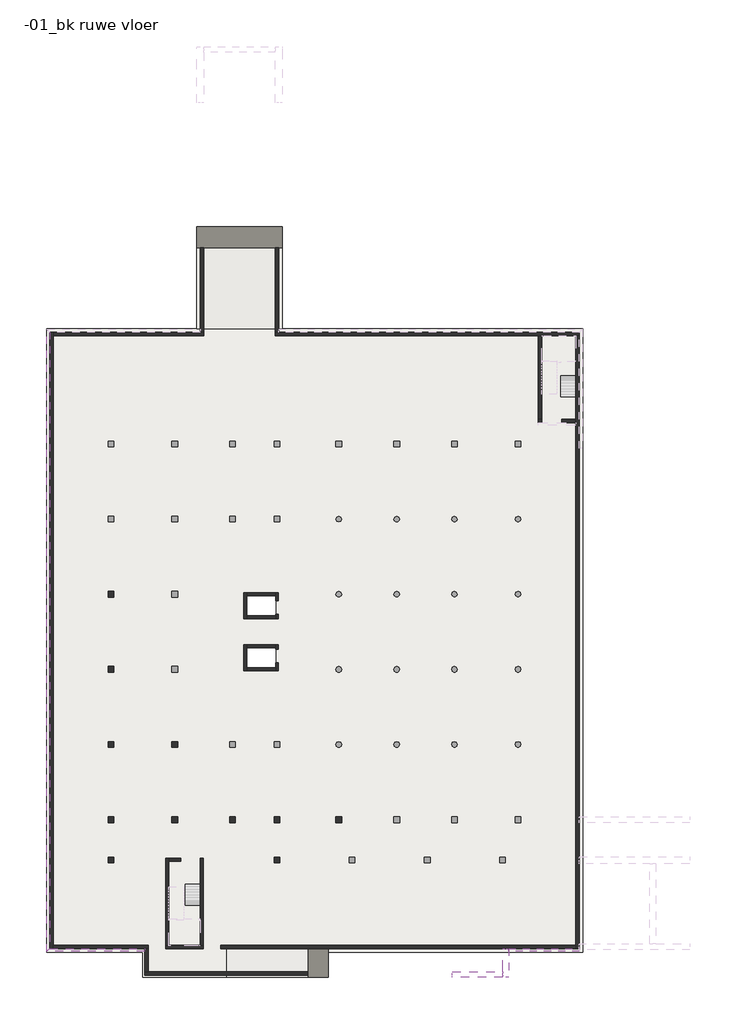
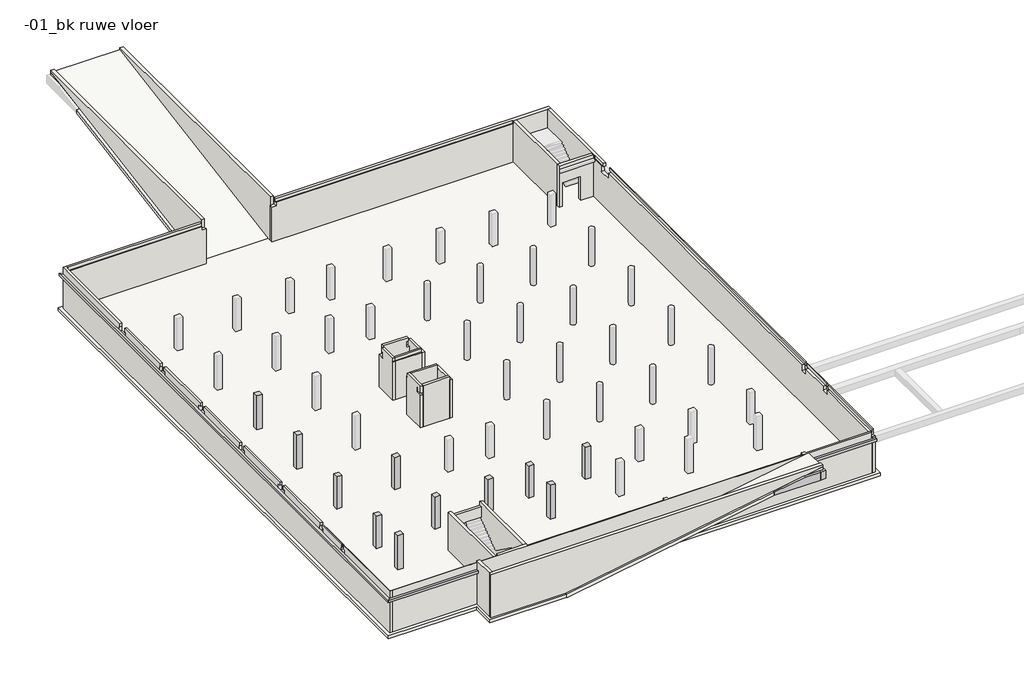
# One storey, part 1 of 2: 22 walls, 15 slabs, 11 columns, 5 beams.
"""IFC4 building model written with IfcOpenShell, lengths in millimetres."""

from ifc_helpers import new_model, si_unit, frame, origin, place, context, project, spatial, polyline, outline, extrude, faceted_brep, element, save

model = new_model("IFC4")

# Units and contexts
model_context = context("Model", 3, world=origin())
ifc_project = project(units=[si_unit("LENGTHUNIT", "METRE", prefix="MILLI")], contexts=[model_context])

# Site, building, storey
site = spatial("IfcSite", under=ifc_project)
building = spatial("IfcBuilding", under=site)
storey = spatial("IfcBuildingStorey", under=building, Name="-01_bk ruwe vloer", Elevation=-4200.0)

# Beams
placement = place(None, origin())
element("IfcBeam", 1, ObjectType="NLRS_16_SF_LIB_oplegnok beton prefab framing-CWV-MMBPC-SRP_gen_rsf : oplegnok beton prefab_gen__bxh 250x250/220", at=placement, inside=storey, context=model_context, shape_type="Brep", body=[
    faceted_brep([(6100.0, 53400.0, -970.0), (6100.0, -400.0, -970.0), (6100.0, -400.0, -750.0), (6100.0, 53400.0, -750.0), (6350.0, 53150.0, -1000.0), (6350.0, -150.0, -1000.0), (6350.0, -150.0, -750.0), (6350.0, 53150.0, -750.0)], [[[0, 1, 2, 3]], [[1, 0, 4, 5]], [[3, 2, 6, 7]], [[5, 4, 7, 6]], [[0, 3, 7, 4]], [[2, 1, 5, 6]]]),
])
element("IfcBeam", 2, ObjectType="NLRS_16_SF_LIB_oplegnok beton prefab framing-CWV-MMBPC-SRP_gen_rsf : oplegnok beton prefab_gen__bxh 250x250/220", at=placement, inside=storey, context=model_context, shape_type="Brep", body=[
    faceted_brep([(14575.0, -400.0, -750.0), (14575.0, -400.0, -970.0), (14575.0, -150.0, -1000.0), (14575.0, -150.0, -750.0), (6100.0, -400.0, -970.0), (6100.0, -400.0, -750.0), (6350.0, -150.0, -1000.0), (6350.0, -150.0, -750.0)], [[[0, 1, 2, 3]], [[4, 1, 0, 5]], [[6, 2, 1, 4]], [[7, 3, 2, 6]], [[5, 0, 3, 7]], [[5, 7, 6, 4]]]),
])
element("IfcBeam", 3, ObjectType="NLRS_16_SF_LIB_funderingsbalk beton ihwg-CWV-MMBC-SRP_gen_rsf : funderingsbalk beton ihwg_gen__bxh 500x800", at=placement, inside=storey, context=model_context, shape_type="Brep", body=[
    faceted_brep([(45545.0, -2650.0, -370.0), (46045.0, -2650.0, -370.0), (46045.0, -150.0, -370.0), (45845.0, -150.0, -370.0), (45845.0, -2450.0, -370.0), (45545.0, -2450.0, -370.0), (46045.0, -2650.0, -1170.0), (46045.0, -150.0, -1170.0), (45545.0, -2650.0, -1170.0), (45545.0, -2150.0, -1170.0), (45545.0, -150.0, -1170.0), (45545.0, -2450.0, -425.486389), (45545.0, -2150.0, -425.486389), (45545.0, -150.0, -425.486389), (45845.0, -150.0, -374.3303196), (45845.0, -2450.0, -374.3303196)], [[[0, 1, 2, 3, 4, 5]], [[1, 6, 7, 2]], [[6, 8, 9, 10, 7]], [[8, 0, 5, 11, 12, 13, 10, 9]], [[1, 0, 8, 6]], [[2, 7, 10, 13, 14, 3]], [[15, 14, 13, 12, 11]], [[14, 15, 4, 3]], [[15, 11, 5, 4]]]),
])
element("IfcBeam", 4, ObjectType="NLRS_16_SF_LIB_funderingsbalk beton ihwg-CWV-MMBC-SRP_gen_rsf : funderingsbalk beton ihwg_gen__bxh 500x800", at=placement, inside=storey, context=model_context, shape_type="Brep", body=[
    faceted_brep([(41178.8693319, -2650.0, -1170.0), (41178.8693319, -2650.0, -865.6696804), (41178.8693319, -2450.0, -865.6696804), (41178.8693319, -2450.0, -1170.0), (44085.6779661, -2650.0, -370.0), (45545.0, -2650.0, -370.0), (45545.0, -2450.0, -370.0), (44085.6779661, -2450.0, -370.0), (45545.0, -2650.0, -1170.0), (45545.0, -2150.0, -1170.0), (41178.8693319, -2150.0, -1170.0), (45545.0, -2150.0, -425.486389), (45545.0, -2450.0, -425.486389)], [[[0, 1, 2, 3]], [[4, 5, 6, 7]], [[1, 0, 8, 5, 4]], [[9, 8, 0, 3, 10]], [[9, 10, 11]], [[8, 9, 11, 12, 6, 5]], [[1, 4, 7, 2]], [[3, 12, 11, 10]], [[12, 3, 2, 7, 6]]]),
])
element("IfcBeam", 5, ObjectType="NLRS_16_SF_LIB_oplegnok beton prefab framing-CWV-MMBPC-SRP_gen_rsf : oplegnok beton prefab_gen__bxh 250x250/220", at=placement, inside=storey, context=model_context, shape_type="SweptSolid", body=[
    extrude(outline(polyline([(-400.0, -750.0), (-150.0, -750.0), (-150.0, -1000.0), (-400.0, -970.0), (-400.0, -750.0)])), frame((46045.0, 0.0, 0.0), z_axis=(1.0, 0.0, 0.0), x_axis=(0.0, 1.0, 0.0)), (0.0, 0.0, 1.0), 6105.0),
])

# Columns
element("IfcColumn", 6, ObjectType="NLRS_28_SCO_TLB_vierkante kolom beton prefab-BCPG-MMBPC-SRP_gen_rsf : kolom vierkant beton prefab_gen__bxh 500x500", at=placement, inside=storey, context=model_context, shape_type="SweptSolid", body=[
    extrude(outline(polyline([(26250.0, 7750.0), (26250.0, 7250.0), (25750.0, 7250.0), (25750.0, 7750.0), (26250.0, 7750.0)])), frame((0.0, 0.0, -4170.0), z_axis=(0.0, 0.0, 1.0), x_axis=(1.0, 0.0, 0.0)), (0.0, 0.0, 1.0), 3400.0),
])
element("IfcColumn", 7, ObjectType="NLRS_28_SCO_TLB_vierkante kolom beton prefab-BCPG-MMBPC-SRP_gen_rsf : kolom vierkant beton prefab_gen__bxh 500x500", at=placement, inside=storey, context=model_context, shape_type="SweptSolid", body=[
    extrude(outline(polyline([(31600.0, 11250.0), (31600.0, 10750.0), (31100.0, 10750.0), (31100.0, 11250.0), (31600.0, 11250.0)])), frame((0.0, 0.0, -4170.0), z_axis=(0.0, 0.0, 1.0), x_axis=(1.0, 0.0, 0.0)), (0.0, 0.0, 1.0), 3200.0),
])
element("IfcColumn", 8, ObjectType="NLRS_28_SCO_TLB_vierkante kolom beton prefab-BCPG-MMBPC-SRP_gen_rsf : kolom vierkant beton prefab_gen__bxh 500x500", at=placement, inside=storey, context=model_context, shape_type="SweptSolid", body=[
    extrude(outline(polyline([(26250.0, 11250.0), (26250.0, 10750.0), (25750.0, 10750.0), (25750.0, 11250.0), (26250.0, 11250.0)])), frame((0.0, 0.0, -4170.0), z_axis=(0.0, 0.0, 1.0), x_axis=(1.0, 0.0, 0.0)), (0.0, 0.0, 1.0), 3200.0),
])
element("IfcColumn", 9, ObjectType="NLRS_28_SCO_TLB_vierkante kolom beton prefab-BCPG-MMBPC-SRP_gen_rsf : kolom vierkant beton prefab_gen__bxh 500x500", at=placement, inside=storey, context=model_context, shape_type="SweptSolid", body=[
    extrude(outline(polyline([(17400.0, 11250.0), (17400.0, 10750.0), (16900.0, 10750.0), (16900.0, 11250.0), (17400.0, 11250.0)])), frame((0.0, 0.0, -4170.0), z_axis=(0.0, 0.0, 1.0), x_axis=(1.0, 0.0, 0.0)), (0.0, 0.0, 1.0), 3200.0),
])
element("IfcColumn", 10, ObjectType="NLRS_28_SCO_TLB_vierkante kolom beton prefab-BCPG-MMBPC-SRP_gen_rsf : kolom vierkant beton prefab_gen__bxh 500x500", at=placement, inside=storey, context=model_context, shape_type="SweptSolid", body=[
    extrude(outline(polyline([(17400.0, 17750.0), (17400.0, 17250.0), (16900.0, 17250.0), (16900.0, 17750.0), (17400.0, 17750.0)])), frame((0.0, 0.0, -4170.0), z_axis=(0.0, 0.0, 1.0), x_axis=(1.0, 0.0, 0.0)), (0.0, 0.0, 1.0), 3200.0),
])
element("IfcColumn", 11, ObjectType="NLRS_28_SCO_TLB_vierkante kolom beton prefab-BCPG-MMBPC-SRP_gen_rsf : kolom vierkant beton prefab_gen__bxh 500x500", at=placement, inside=storey, context=model_context, shape_type="SweptSolid", body=[
    extrude(outline(polyline([(11900.0, 11250.0), (11900.0, 10750.0), (11400.0, 10750.0), (11400.0, 11250.0), (11900.0, 11250.0)])), frame((0.0, 0.0, -4170.0), z_axis=(0.0, 0.0, 1.0), x_axis=(1.0, 0.0, 0.0)), (0.0, 0.0, 1.0), 3200.0),
])
element("IfcColumn", 12, ObjectType="NLRS_28_SCO_TLB_vierkante kolom beton prefab-BCPG-MMBPC-SRP_gen_rsf : kolom vierkant beton prefab_gen__bxh 500x500", at=placement, inside=storey, context=model_context, shape_type="SweptSolid", body=[
    extrude(outline(polyline([(11900.0, 17750.0), (11900.0, 17250.0), (11400.0, 17250.0), (11400.0, 17750.0), (11900.0, 17750.0)])), frame((0.0, 0.0, -4170.0), z_axis=(0.0, 0.0, 1.0), x_axis=(1.0, 0.0, 0.0)), (0.0, 0.0, 1.0), 3200.0),
])
element("IfcColumn", 13, ObjectType="NLRS_28_SCO_TLB_vierkante kolom beton prefab-BCPG-MMBPC-SRP_gen_rsf : kolom vierkant beton prefab_gen__bxh 500x500", at=placement, inside=storey, context=model_context, shape_type="SweptSolid", body=[
    extrude(outline(polyline([(11900.0, 24250.0), (11900.0, 23750.0), (11400.0, 23750.0), (11400.0, 24250.0), (11900.0, 24250.0)])), frame((0.0, 0.0, -4170.0), z_axis=(0.0, 0.0, 1.0), x_axis=(1.0, 0.0, 0.0)), (0.0, 0.0, 1.0), 3400.0),
])
element("IfcColumn", 14, ObjectType="NLRS_28_SCO_TLB_vierkante kolom beton prefab-BCPG-MMBPC-SRP_gen_rsf : kolom vierkant beton prefab_gen__bxh 500x500", at=placement, inside=storey, context=model_context, shape_type="SweptSolid", body=[
    extrude(outline(polyline([(11900.0, 30750.0), (11900.0, 30250.0), (11400.0, 30250.0), (11400.0, 30750.0), (11900.0, 30750.0)])), frame((0.0, 0.0, -4170.0), z_axis=(0.0, 0.0, 1.0), x_axis=(1.0, 0.0, 0.0)), (0.0, 0.0, 1.0), 3400.0),
])
element("IfcColumn", 15, ObjectType="NLRS_28_SCO_TLB_vierkante kolom beton prefab-BCPG-MMBPC-SRP_gen_rsf : kolom vierkant beton prefab_gen__bxh 500x500", at=placement, inside=storey, context=model_context, shape_type="SweptSolid", body=[
    extrude(outline(polyline([(11900.0, 7750.0), (11900.0, 7250.0), (11400.0, 7250.0), (11400.0, 7750.0), (11900.0, 7750.0)])), frame((0.0, 0.0, -4170.0), z_axis=(0.0, 0.0, 1.0), x_axis=(1.0, 0.0, 0.0)), (0.0, 0.0, 1.0), 3400.0),
])
element("IfcColumn", 16, ObjectType="NLRS_28_SCO_TLB_vierkante kolom beton prefab-BCPG-MMBPC-SRP_gen_rsf : kolom vierkant beton prefab_gen__bxh 500x500", at=placement, inside=storey, context=model_context, shape_type="SweptSolid", body=[
    extrude(outline(polyline([(22400.0, 11250.0), (22400.0, 10750.0), (21900.0, 10750.0), (21900.0, 11250.0), (22400.0, 11250.0)])), frame((0.0, 0.0, -4170.0), z_axis=(0.0, 0.0, 1.0), x_axis=(1.0, 0.0, 0.0)), (0.0, 0.0, 1.0), 3200.0),
])

# Slabs
element("IfcSlab", 17, ObjectType="NLRS_13_FL_beton ihwg 300_gen_rsf", at=placement, inside=storey, context=model_context, shape_type="Brep", body=[
    faceted_brep([(6070.0, 53450.0, -4500.0), (48305.0, 53450.0, -4500.0), (52450.0, 53450.0, -4500.0), (52450.0, 45050.0, -4500.0), (52450.0, -450.0, -4500.0), (21650.3947557, -450.0, -4500.0), (21625.0, -450.0, -4500.0), (21625.0, -2650.0, -4500.0), (14375.0, -2650.0, -4500.0), (14375.0, -450.0, -4500.0), (6070.0, -450.0, -4500.0), (25875.0, 30375.0, -4500.0), (23375.0, 30375.0, -4500.0), (23375.0, 28625.0, -4500.0), (25875.0, 28625.0, -4500.0), (25875.0, 25875.0, -4500.0), (23375.0, 25875.0, -4500.0), (23375.0, 24125.0, -4500.0), (25875.0, 24125.0, -4500.0), (6070.0, 53450.0, -4200.0), (6070.0, -450.0, -4200.0), (14375.0, -450.0, -4200.0), (14375.0, -2650.0, -4200.0), (21625.0, -2650.0, -4200.0), (21625.0, -450.0, -4200.0), (23409.7167896, -450.0, -4200.0), (52450.0, -450.0, -4200.0), (52450.0, 53450.0, -4200.0), (25875.0, 25875.0, -4200.0), (25875.0, 25752.0, -4200.0), (25875.0, 24552.0, -4200.0), (25875.0, 24125.0, -4200.0), (23375.0, 24125.0, -4200.0), (23375.0, 25875.0, -4200.0), (25875.0, 30375.0, -4200.0), (25875.0, 29948.0, -4200.0), (25875.0, 28748.0, -4200.0), (25875.0, 28625.0, -4200.0), (23375.0, 28625.0, -4200.0), (23375.0, 30375.0, -4200.0)], [[[0, 1, 2, 3, 4, 5, 6, 7, 8, 9, 10], [11, 12, 13, 14], [15, 16, 17, 18]], [[19, 20, 21, 22, 23, 24, 25, 26, 27], [28, 29, 30, 31, 32, 33], [34, 35, 36, 37, 38, 39]], [[4, 3, 2, 27, 26]], [[6, 5, 4, 26, 25, 24]], [[0, 10, 20, 19]], [[7, 6, 24, 23]], [[8, 7, 23, 22]], [[9, 8, 22, 21]], [[10, 9, 21, 20]], [[2, 1, 0, 19, 27]], [[12, 11, 34, 39]], [[13, 12, 39, 38]], [[14, 13, 38, 37]], [[11, 14, 37, 36, 35, 34]], [[16, 15, 28, 33]], [[17, 16, 33, 32]], [[18, 17, 32, 31]], [[15, 18, 31, 30, 29, 28]]]),
])
element("IfcSlab", 18, ObjectType="NLRS_13_FL_beton ihwg 300_gen_rsf", at=placement, inside=storey, context=model_context, shape_type="Brep", body=[
    faceted_brep([(19050.0, 53450.0, -4504.3303196), (19050.0, 73003.8693319, -1170.0), (19350.0, 73003.8693319, -1170.0), (19350.0, 77670.0, -374.3303196), (19650.0, 77670.0, -374.3303196), (25850.0, 77670.0, -374.3303196), (26150.0, 77670.0, -374.3303196), (26150.0, 73003.8693319, -1170.0), (26450.0, 73003.8693319, -1170.0), (26450.0, 53450.0, -4504.3303196), (19050.0, 53450.0, -4200.0), (26450.0, 53450.0, -4200.0), (26450.0, 73003.8693319, -865.6696804), (26150.0, 73003.8693319, -865.6696804), (26150.0, 75910.6779661, -370.0), (26150.0, 77670.0, -70.0), (25850.0, 77670.0, -70.0), (19650.0, 77670.0, -70.0), (19350.0, 77670.0, -70.0), (19350.0, 75910.6779661, -370.0), (19350.0, 73003.8693319, -865.6696804), (19050.0, 73003.8693319, -865.6696804), (19350.0, 77670.0, -370.0), (26150.0, 77670.0, -370.0)], [[[0, 1, 2, 3, 4, 5, 6, 7, 8, 9]], [[10, 11, 12, 13, 14, 15, 16, 17, 18, 19, 20, 21]], [[1, 0, 10, 21]], [[6, 5, 4, 3, 22, 18, 17, 16, 15, 23]], [[9, 8, 12, 11]], [[0, 9, 11, 10]], [[2, 1, 21, 20]], [[3, 2, 20, 19, 18, 22]], [[7, 6, 23, 15, 14, 13]], [[8, 7, 13, 12]]]),
])
element("IfcSlab", 19, ObjectType="NLRS_13_FL_beton ihwg 300_gen_rsf", at=placement, inside=storey, context=model_context, shape_type="Brep", body=[
    faceted_brep([(45845.0, -150.0, -374.3303196), (45845.0, -2450.0, -374.3303196), (45545.0, -2450.0, -425.486389), (41178.8693319, -2450.0, -1170.0), (41178.8693319, -2650.0, -1170.0), (21625.0, -2650.0, -4504.3303196), (21625.0, -150.0, -4504.3303196), (21650.3947557, -150.0, -4500.0), (21650.3947557, -450.0, -4500.0), (23409.7167896, -450.0, -4200.0), (23409.7167896, -150.0, -4200.0), (45545.0, -150.0, -425.486389), (45845.0, -2450.0, -70.0), (45845.0, -2150.0, -70.0), (45845.0, -150.0, -70.0), (21625.0, -150.0, -4200.0), (21625.0, -450.0, -4200.0), (21625.0, -2650.0, -4200.0), (41178.8693319, -2650.0, -865.6696804), (41178.8693319, -2450.0, -865.6696804), (44085.6779661, -2450.0, -370.0), (45845.0, -150.0, -370.0), (45845.0, -2450.0, -370.0), (21625.0, -2650.0, -4500.0), (21625.0, -450.0, -4500.0), (21625.0, -150.0, -4500.0)], [[[0, 1, 2, 3, 4, 5, 6, 7, 8, 9, 10, 11]], [[12, 13, 14, 15, 16, 17, 18, 19, 20]], [[1, 0, 21, 14, 13, 12, 22]], [[5, 4, 18, 17, 23]], [[6, 5, 23, 17, 16, 24, 25]], [[15, 14, 21, 0, 11, 10]], [[7, 6, 25]], [[24, 8, 7, 25]], [[9, 16, 15, 10]], [[8, 24, 16, 9]], [[3, 2, 1, 22, 12, 20, 19]], [[4, 3, 19, 18]]]),
])
element("IfcSlab", 20, ObjectType="NLRS_16_SFO_LB_funderingspoer meerpaals beton ihwg-MMBC-SH_gen_rsf : funderingspoer beton ihwg_gen__4-paals bxlxh 1800x1800x1200", at=placement, inside=storey, context=model_context, shape_type="SweptSolid", body=[
    extrude(outline(polyline([(16250.0, 16600.0), (16250.0, 18400.0), (18050.0, 18400.0), (18050.0, 16600.0), (16250.0, 16600.0)])), frame((0.0, 0.0, -5400.0), z_axis=(0.0, 0.0, 1.0), x_axis=(1.0, 0.0, 0.0)), (0.0, 0.0, 1.0), 900.0),
])
element("IfcSlab", 21, ObjectType="NLRS_16_SFO_LB_funderingspoer meerpaals beton ihwg-MMBC-SH_gen_rsf : funderingspoer beton ihwg_gen__3-paals bxlxh 1800x1800x1200", at=placement, inside=storey, context=model_context, shape_type="SweptSolid", body=[
    extrude(outline(polyline([(18050.0, 12075.0), (18050.0, 10275.0), (16250.0, 10275.0), (16250.0, 12075.0), (18050.0, 12075.0)])), frame((0.0, 0.0, -5400.0), z_axis=(0.0, 0.0, 1.0), x_axis=(1.0, 0.0, 0.0)), (0.0, 0.0, 1.0), 900.0),
])
element("IfcSlab", 22, ObjectType="NLRS_16_SFO_LB_funderingspoer meerpaals beton ihwg-MMBC-SH_gen_rsf : funderingspoer beton ihwg_gen__2-paals bxlxh 700x1800x1200", at=placement, inside=storey, context=model_context, shape_type="SweptSolid", body=[
    extrude(outline(polyline([(11300.0, 31400.0), (12000.0, 31400.0), (12000.0, 29600.0), (11300.0, 29600.0), (11300.0, 31400.0)])), frame((0.0, 0.0, -5400.0), z_axis=(0.0, 0.0, 1.0), x_axis=(1.0, 0.0, 0.0)), (0.0, 0.0, 1.0), 900.0),
])
element("IfcSlab", 23, ObjectType="NLRS_16_SFO_LB_funderingspoer meerpaals beton ihwg-MMBC-SH_gen_rsf : funderingspoer beton ihwg_gen__2-paals bxlxh 700x1800x1200", at=placement, inside=storey, context=model_context, shape_type="SweptSolid", body=[
    extrude(outline(polyline([(11300.0, 24900.0), (12000.0, 24900.0), (12000.0, 23100.0), (11300.0, 23100.0), (11300.0, 24900.0)])), frame((0.0, 0.0, -5400.0), z_axis=(0.0, 0.0, 1.0), x_axis=(1.0, 0.0, 0.0)), (0.0, 0.0, 1.0), 900.0),
])
element("IfcSlab", 24, ObjectType="NLRS_16_SFO_LB_funderingspoer meerpaals beton ihwg-MMBC-SH_gen_rsf : funderingspoer beton ihwg_gen__2-paals bxlxh 700x1800x1200", at=placement, inside=storey, context=model_context, shape_type="SweptSolid", body=[
    extrude(outline(polyline([(11300.0, 18400.0), (12000.0, 18400.0), (12000.0, 16600.0), (11300.0, 16600.0), (11300.0, 18400.0)])), frame((0.0, 0.0, -5400.0), z_axis=(0.0, 0.0, 1.0), x_axis=(1.0, 0.0, 0.0)), (0.0, 0.0, 1.0), 900.0),
])
element("IfcSlab", 25, ObjectType="NLRS_16_SFO_LB_funderingspoer meerpaals beton ihwg-MMBC-SH_gen_rsf : funderingspoer beton ihwg_gen__1-paals bxlxh 700x700x500", at=placement, inside=storey, context=model_context, shape_type="SweptSolid", body=[
    extrude(outline(polyline([(11300.0, 11350.0), (12000.0, 11350.0), (12000.0, 10650.0), (11300.0, 10650.0), (11300.0, 11350.0)])), frame((0.0, 0.0, -4700.0), z_axis=(0.0, 0.0, 1.0), x_axis=(1.0, 0.0, 0.0)), (0.0, 0.0, 1.0), 200.0),
])
element("IfcSlab", 26, ObjectType="NLRS_16_SFO_LB_funderingspoer meerpaals beton ihwg-MMBC-SH_gen_rsf : funderingspoer beton ihwg_gen__1-paals bxlxh 700x700x500", at=placement, inside=storey, context=model_context, shape_type="SweptSolid", body=[
    extrude(outline(polyline([(11300.0, 7850.0), (12000.0, 7850.0), (12000.0, 7150.0), (11300.0, 7150.0), (11300.0, 7850.0)])), frame((0.0, 0.0, -4700.0), z_axis=(0.0, 0.0, 1.0), x_axis=(1.0, 0.0, 0.0)), (0.0, 0.0, 1.0), 200.0),
])
element("IfcSlab", 27, ObjectType="NLRS_16_SFO_LB_funderingspoer meerpaals beton ihwg-MMBC-SH_gen_rsf : funderingspoer beton ihwg_gen__1-paals bxlxh 700x700x500", at=placement, inside=storey, context=model_context, shape_type="SweptSolid", body=[
    extrude(outline(polyline([(21800.0, 11350.0), (22500.0, 11350.0), (22500.0, 10650.0), (21800.0, 10650.0), (21800.0, 11350.0)])), frame((0.0, 0.0, -4700.0), z_axis=(0.0, 0.0, 1.0), x_axis=(1.0, 0.0, 0.0)), (0.0, 0.0, 1.0), 200.0),
])
element("IfcSlab", 28, ObjectType="NLRS_16_SFO_LB_funderingspoer meerpaals beton ihwg-MMBC-SH_gen_rsf : funderingspoer beton ihwg_gen__2-paals bxlxh 700x1800x1200", at=placement, inside=storey, context=model_context, shape_type="SweptSolid", body=[
    extrude(outline(polyline([(31000.0, 11900.0), (31700.0, 11900.0), (31700.0, 10100.0), (31000.0, 10100.0), (31000.0, 11900.0)])), frame((0.0, 0.0, -5400.0), z_axis=(0.0, 0.0, 1.0), x_axis=(1.0, 0.0, 0.0)), (0.0, 0.0, 1.0), 900.0),
])
element("IfcSlab", 29, ObjectType="NLRS_16_SFO_LB_funderingspoer meerpaals beton ihwg-MMBC-SH_gen_rsf : funderingspoer beton ihwg_gen__4-paals bxlxh 1800x1800x1200", at=placement, inside=storey, context=model_context, shape_type="SweptSolid", body=[
    extrude(outline(polyline([(25100.0, 6600.0), (25100.0, 8400.0), (26900.0, 8400.0), (26900.0, 6600.0), (25100.0, 6600.0)])), frame((0.0, 0.0, -5400.0), z_axis=(0.0, 0.0, 1.0), x_axis=(1.0, 0.0, 0.0)), (0.0, 0.0, 1.0), 900.0),
])
element("IfcSlab", 30, ObjectType="NLRS_16_SFO_LB_funderingspoer meerpaals beton ihwg-MMBC-SH_gen_rsf : funderingspoer beton ihwg_gen__trap bxlxh 3800x9300x1200", at=placement, inside=storey, context=model_context, shape_type="SweptSolid", body=[
    extrude(outline(polyline([(19900.0, -900.0), (16100.0, -900.0), (16100.0, 8400.0), (19900.0, 8400.0), (19900.0, -900.0)])), frame((0.0, 0.0, -5400.0), z_axis=(0.0, 0.0, 1.0), x_axis=(1.0, 0.0, 0.0)), (0.0, 0.0, 1.0), 900.0),
])
element("IfcSlab", 31, ObjectType="NLRS_16_SFO_LB_funderingspoer meerpaals beton ihwg-MMBC-SH_gen_rsf : funderingspoer beton ihwg_gen__3-paals bxlxh 1800x1800x1200", at=placement, inside=storey, context=model_context, shape_type="SweptSolid", body=[
    extrude(outline(polyline([(26900.0, 12075.0), (26900.0, 10275.0), (25100.0, 10275.0), (25100.0, 12075.0), (26900.0, 12075.0)])), frame((0.0, 0.0, -5400.0), z_axis=(0.0, 0.0, 1.0), x_axis=(1.0, 0.0, 0.0)), (0.0, 0.0, 1.0), 900.0),
])

# Walls
element("IfcWall", 32, ObjectType="NLRS_16_WA_hollewand 300_gen_rsf", at=placement, inside=storey, context=model_context, shape_type="Brep", body=[
    faceted_brep([(6650.0, -150.0, -4200.0), (6650.0, 150.0, -4200.0), (6650.0, 52850.0, -4200.0), (6650.0, 53150.0, -4200.0), (6650.0, 53150.0, -70.0), (6650.0, 52950.0, -70.0), (6650.0, 52950.0, -390.0), (6650.0, 52850.0, -390.0), (6650.0, 44100.0, -390.0), (6650.0, 44100.0, -970.0), (6650.0, 42900.0, -970.0), (6650.0, 42900.0, -390.0), (6650.0, 37500.0, -390.0), (6650.0, 37500.0, -970.0), (6650.0, 36500.0, -970.0), (6650.0, 36500.0, -390.0), (6650.0, 31000.0, -390.0), (6650.0, 31000.0, -970.0), (6650.0, 30000.0, -970.0), (6650.0, 30000.0, -390.0), (6650.0, 24500.0, -390.0), (6650.0, 24500.0, -970.0), (6650.0, 23500.0, -970.0), (6650.0, 23500.0, -390.0), (6650.0, 18000.0, -390.0), (6650.0, 18000.0, -970.0), (6650.0, 17000.0, -970.0), (6650.0, 17000.0, -390.0), (6650.0, 11350.0, -390.0), (6650.0, 11350.0, -970.0), (6650.0, 10650.0, -970.0), (6650.0, 10650.0, -390.0), (6650.0, 7850.0, -390.0), (6650.0, 7850.0, -770.0), (6650.0, 7150.0, -770.0), (6650.0, 7150.0, -390.0), (6650.0, 150.0, -390.0), (6650.0, -90.0, -390.0), (6650.0, -90.0, -70.0), (6650.0, -150.0, -70.0), (6350.0, 53150.0, -4200.0), (6350.0, -150.0, -4200.0), (6350.0, -150.0, -70.0), (6350.0, 7350.0, -70.0), (6350.0, 7350.0, -390.0), (6350.0, 7150.0, -390.0), (6350.0, 7150.0, -770.0), (6350.0, 7850.0, -770.0), (6350.0, 7850.0, -390.0), (6350.0, 7650.0, -390.0), (6350.0, 7650.0, -70.0), (6350.0, 10850.0, -70.0), (6350.0, 10850.0, -390.0), (6350.0, 10650.0, -390.0), (6350.0, 10650.0, -970.0), (6350.0, 11350.0, -970.0), (6350.0, 11350.0, -390.0), (6350.0, 11150.0, -390.0), (6350.0, 11150.0, -70.0), (6350.0, 17200.0, -70.0), (6350.0, 17200.0, -390.0), (6350.0, 17000.0, -390.0), (6350.0, 17000.0, -970.0), (6350.0, 18000.0, -970.0), (6350.0, 18000.0, -390.0), (6350.0, 17800.0, -390.0), (6350.0, 17800.0, -70.0), (6350.0, 23700.0, -70.0), (6350.0, 23700.0, -390.0), (6350.0, 23500.0, -390.0), (6350.0, 23500.0, -970.0), (6350.0, 24500.0, -970.0), (6350.0, 24500.0, -390.0), (6350.0, 24300.0, -390.0), (6350.0, 24300.0, -70.0), (6350.0, 30200.0, -70.0), (6350.0, 30200.0, -390.0), (6350.0, 30000.0, -390.0), (6350.0, 30000.0, -970.0), (6350.0, 31000.0, -970.0), (6350.0, 31000.0, -390.0), (6350.0, 30800.0, -390.0), (6350.0, 30800.0, -70.0), (6350.0, 36700.0, -70.0), (6350.0, 36700.0, -390.0), (6350.0, 36500.0, -390.0), (6350.0, 36500.0, -970.0), (6350.0, 37500.0, -970.0), (6350.0, 37500.0, -390.0), (6350.0, 37300.0, -390.0), (6350.0, 37300.0, -70.0), (6350.0, 43100.0, -70.0), (6350.0, 43100.0, -390.0), (6350.0, 42900.0, -390.0), (6350.0, 42900.0, -970.0), (6350.0, 44100.0, -970.0), (6350.0, 44100.0, -390.0), (6350.0, 43900.0, -390.0), (6350.0, 43900.0, -70.0), (6350.0, 53150.0, -70.0), (6410.0, -90.0, -70.0), (6410.0, 7350.0, -70.0), (6410.0, 7650.0, -70.0), (6410.0, 10850.0, -70.0), (6550.0, 17800.0, -70.0), (6550.0, 23700.0, -70.0), (6550.0, 24300.0, -70.0), (6550.0, 30200.0, -70.0), (6550.0, 30800.0, -70.0), (6550.0, 36700.0, -70.0), (6550.0, 37300.0, -70.0), (6550.0, 43100.0, -70.0), (6550.0, 43900.0, -70.0), (6550.0, 52950.0, -70.0), (6550.0, 11150.0, -70.0), (6550.0, 17200.0, -70.0), (6410.0, -90.0, -390.0), (6410.0, 7150.0, -390.0), (6410.0, 7350.0, -390.0), (6550.0, 17200.0, -390.0), (6550.0, 17800.0, -390.0), (6550.0, 23700.0, -390.0), (6550.0, 24300.0, -390.0), (6550.0, 30200.0, -390.0), (6550.0, 30800.0, -390.0), (6550.0, 36700.0, -390.0), (6550.0, 37300.0, -390.0), (6550.0, 43100.0, -390.0), (6550.0, 42900.0, -390.0), (6550.0, 44100.0, -390.0), (6550.0, 43900.0, -390.0), (6550.0, 36500.0, -390.0), (6550.0, 37500.0, -390.0), (6550.0, 30000.0, -390.0), (6550.0, 31000.0, -390.0), (6550.0, 23500.0, -390.0), (6550.0, 24500.0, -390.0), (6550.0, 17000.0, -390.0), (6550.0, 18000.0, -390.0), (6410.0, 10650.0, -390.0), (6410.0, 7850.0, -390.0), (6410.0, 7650.0, -390.0), (6410.0, 10850.0, -390.0), (6550.0, 11350.0, -390.0), (6550.0, 11150.0, -390.0), (6550.0, 52950.0, -390.0)], [[[0, 1, 2, 3, 4, 5, 6, 7, 8, 9, 10, 11, 12, 13, 14, 15, 16, 17, 18, 19, 20, 21, 22, 23, 24, 25, 26, 27, 28, 29, 30, 31, 32, 33, 34, 35, 36, 37, 38, 39]], [[40, 41, 42, 43, 44, 45, 46, 47, 48, 49, 50, 51, 52, 53, 54, 55, 56, 57, 58, 59, 60, 61, 62, 63, 64, 65, 66, 67, 68, 69, 70, 71, 72, 73, 74, 75, 76, 77, 78, 79, 80, 81, 82, 83, 84, 85, 86, 87, 88, 89, 90, 91, 92, 93, 94, 95, 96, 97, 98, 99]], [[3, 2, 1, 0, 41, 40]], [[42, 39, 38, 100, 101, 43]], [[102, 103, 51, 50]], [[67, 66, 104, 105]], [[75, 74, 106, 107]], [[83, 82, 108, 109]], [[91, 90, 110, 111]], [[99, 98, 112, 113, 5, 4]], [[59, 58, 114, 115]], [[0, 39, 42, 41]], [[116, 37, 36, 35, 117]], [[116, 100, 38, 37]], [[100, 116, 117, 118, 101]], [[59, 115, 119, 60]], [[104, 66, 65, 120]], [[67, 105, 121, 68]], [[106, 74, 73, 122]], [[75, 107, 123, 76]], [[108, 82, 81, 124]], [[83, 109, 125, 84]], [[110, 90, 89, 126]], [[92, 91, 111, 127]], [[93, 92, 127, 128]], [[10, 94, 93, 128, 11]], [[94, 10, 9, 95]], [[95, 9, 8, 129, 96]], [[97, 96, 129, 130]], [[98, 97, 130, 112]], [[14, 86, 85, 131, 15]], [[86, 14, 13, 87]], [[87, 13, 12, 132, 88]], [[89, 88, 132, 126]], [[85, 84, 125, 131]], [[19, 18, 78, 77, 133]], [[17, 79, 78, 18]], [[79, 17, 16, 134, 80]], [[81, 80, 134, 124]], [[77, 76, 123, 133]], [[22, 70, 69, 135, 23]], [[70, 22, 21, 71]], [[71, 21, 20, 136, 72]], [[73, 72, 136, 122]], [[69, 68, 121, 135]], [[26, 62, 61, 137, 27]], [[62, 26, 25, 63]], [[63, 25, 24, 138, 64]], [[65, 64, 138, 120]], [[61, 60, 119, 137]], [[31, 139, 140, 32]], [[103, 102, 141, 140, 139, 142]], [[142, 52, 51, 103]], [[52, 142, 139, 53]], [[53, 139, 31, 30, 54]], [[54, 30, 29, 55]], [[55, 29, 28, 143, 56]], [[57, 56, 143, 144]], [[58, 57, 144, 114]], [[145, 129, 8, 7, 6]], [[145, 113, 112, 130, 129]], [[12, 11, 128, 132]], [[111, 110, 126, 132, 128, 127]], [[16, 15, 131, 134]], [[109, 108, 124, 134, 131, 125]], [[20, 19, 133, 136]], [[107, 106, 122, 136, 133, 123]], [[24, 23, 135, 138]], [[105, 104, 120, 138, 135, 121]], [[28, 27, 137, 143]], [[115, 114, 144, 143, 137, 119]], [[118, 44, 43, 101]], [[44, 118, 117, 45]], [[45, 117, 35, 34, 46]], [[46, 34, 33, 47]], [[140, 48, 47, 33, 32]], [[141, 49, 48, 140]], [[49, 141, 102, 50]], [[4, 3, 40, 99]], [[113, 145, 6, 5]]]),
])
element("IfcWall", 33, ObjectType="NLRS_16_WA_hollewand 300_gen_rsf", at=placement, inside=storey, context=model_context, shape_type="Brep", body=[
    faceted_brep([(6650.0, 52850.0, -4200.0), (19650.0, 52850.0, -4200.0), (19650.0, 52850.0, -720.0), (19250.0, 52850.0, -720.0), (19250.0, 52850.0, -390.0), (6650.0, 52850.0, -390.0), (19650.0, 53150.0, -4200.0), (6650.0, 53150.0, -4200.0), (6650.0, 53150.0, -70.0), (19250.0, 53150.0, -70.0), (19250.0, 53150.0, -720.0), (19650.0, 53150.0, -720.0), (6650.0, 52950.0, -70.0), (19250.0, 52950.0, -70.0), (19250.0, 52950.0, -390.0), (6650.0, 52950.0, -390.0)], [[[0, 1, 2, 3, 4, 5]], [[6, 7, 8, 9, 10, 11]], [[1, 0, 7, 6]], [[1, 6, 11, 2]], [[12, 13, 9, 8]], [[5, 4, 14, 15]], [[13, 12, 15, 14]], [[3, 10, 9, 13, 14, 4]], [[10, 3, 2, 11]], [[8, 7, 0, 5, 15, 12]]]),
])
element("IfcWall", 34, ObjectType="NLRS_16_WA_hollewand 300_gen_rsf", at=placement, inside=storey, context=model_context, shape_type="Brep", body=[
    faceted_brep([(25850.0, 52850.0, -4200.0), (51850.0, 52850.0, -4200.0), (52150.0, 52850.0, -4200.0), (52150.0, 52850.0, -70.0), (51850.0, 52850.0, -70.0), (48605.0, 52850.0, -70.0), (48605.0, 52850.0, -390.0), (26250.0, 52850.0, -390.0), (26250.0, 52850.0, -720.0), (25850.0, 52850.0, -720.0), (52150.0, 53150.0, -4200.0), (25850.0, 53150.0, -4200.0), (25850.0, 53150.0, -720.0), (26250.0, 53150.0, -720.0), (26250.0, 53150.0, -70.0), (52150.0, 53150.0, -70.0), (26250.0, 52950.0, -70.0), (48605.0, 52950.0, -70.0), (48605.0, 52950.0, -390.0), (26250.0, 52950.0, -390.0)], [[[0, 1, 2, 3, 4, 5, 6, 7, 8, 9]], [[10, 11, 12, 13, 14, 15]], [[2, 1, 0, 11, 10]], [[3, 15, 14, 16, 17, 5, 4]], [[11, 0, 9, 12]], [[3, 2, 10, 15]], [[6, 18, 19, 7]], [[18, 6, 5, 17]], [[19, 18, 17, 16]], [[13, 8, 7, 19, 16, 14]], [[8, 13, 12, 9]]]),
])
element("IfcWall", 35, ObjectType="NLRS_16_WA_hollewand 300_gen_rsf", at=placement, inside=storey, context=model_context, shape_type="Brep", body=[
    faceted_brep([(51850.0, 52850.0, -4200.0), (51850.0, 150.0, -4200.0), (51850.0, -150.0, -4200.0), (51850.0, -150.0, -590.0), (51850.0, 150.0, -590.0), (51850.0, 150.0, -390.0), (51850.0, 7150.0, -390.0), (51850.0, 7150.0, -770.0), (51850.0, 7850.0, -770.0), (51850.0, 7850.0, -390.0), (51850.0, 10650.0, -390.0), (51850.0, 10650.0, -970.0), (51850.0, 11350.0, -970.0), (51850.0, 11350.0, -390.0), (51850.0, 42900.0, -390.0), (51850.0, 42900.0, -970.0), (51850.0, 44100.0, -970.0), (51850.0, 44100.0, -390.0), (51850.0, 45270.0, -390.0), (51850.0, 45270.0, -70.0), (51850.0, 52850.0, -70.0), (52150.0, -150.0, -4200.0), (52150.0, 52850.0, -4200.0), (52150.0, 52850.0, -70.0), (52150.0, 43900.0, -70.0), (52150.0, 43900.0, -390.0), (52150.0, 44100.0, -390.0), (52150.0, 44100.0, -970.0), (52150.0, 42900.0, -970.0), (52150.0, 42900.0, -390.0), (52150.0, 43100.0, -390.0), (52150.0, 43100.0, -70.0), (52150.0, 11150.0, -70.0), (52150.0, 11150.0, -390.0), (52150.0, 11350.0, -390.0), (52150.0, 11350.0, -970.0), (52150.0, 10650.0, -970.0), (52150.0, 10650.0, -390.0), (52150.0, 10850.0, -390.0), (52150.0, 10850.0, -70.0), (52150.0, 7650.0, -70.0), (52150.0, 7650.0, -390.0), (52150.0, 7850.0, -390.0), (52150.0, 7850.0, -770.0), (52150.0, 7150.0, -770.0), (52150.0, 7150.0, -390.0), (52150.0, 7350.0, -390.0), (52150.0, 7350.0, -70.0), (52150.0, 150.0, -70.0), (52150.0, 150.0, -590.0), (52150.0, -150.0, -590.0), (51950.0, 45270.0, -70.0), (51950.0, 43900.0, -70.0), (52090.0, 10850.0, -70.0), (52090.0, 7650.0, -70.0), (52090.0, 43100.0, -70.0), (52090.0, 11150.0, -70.0), (52050.0, 7350.0, -70.0), (52050.0, 150.0, -70.0), (52090.0, 43100.0, -390.0), (52090.0, 42900.0, -390.0), (51950.0, 44100.0, -390.0), (51950.0, 43900.0, -390.0), (52090.0, 7850.0, -390.0), (52090.0, 10650.0, -390.0), (52090.0, 10850.0, -390.0), (52090.0, 7650.0, -390.0), (51950.0, 45270.0, -390.0), (52090.0, 11350.0, -390.0), (52090.0, 11150.0, -390.0), (52050.0, 7150.0, -390.0), (52050.0, 150.0, -390.0), (52050.0, 7350.0, -390.0)], [[[0, 1, 2, 3, 4, 5, 6, 7, 8, 9, 10, 11, 12, 13, 14, 15, 16, 17, 18, 19, 20]], [[21, 22, 23, 24, 25, 26, 27, 28, 29, 30, 31, 32, 33, 34, 35, 36, 37, 38, 39, 40, 41, 42, 43, 44, 45, 46, 47, 48, 49, 50]], [[2, 1, 0, 22, 21]], [[23, 20, 19, 51, 52, 24]], [[53, 54, 40, 39]], [[31, 55, 56, 32]], [[47, 57, 58, 48]], [[0, 20, 23, 22]], [[2, 21, 50, 3]], [[31, 30, 59, 55]], [[30, 29, 60, 59]], [[28, 15, 14, 60, 29]], [[15, 28, 27, 16]], [[16, 27, 26, 61, 17]], [[26, 25, 62, 61]], [[25, 24, 52, 62]], [[9, 63, 64, 10]], [[54, 53, 65, 64, 63, 66]], [[61, 67, 18, 17]], [[67, 61, 62, 52, 51]], [[60, 14, 13, 68]], [[56, 55, 59, 60, 68, 69]], [[67, 51, 19, 18]], [[70, 6, 5, 71]], [[57, 72, 70, 71, 58]], [[46, 72, 57, 47]], [[72, 46, 45, 70]], [[70, 45, 44, 7, 6]], [[7, 44, 43, 8]], [[42, 63, 9, 8, 43]], [[63, 42, 41, 66]], [[66, 41, 40, 54]], [[38, 65, 53, 39]], [[65, 38, 37, 64]], [[64, 37, 36, 11, 10]], [[11, 36, 35, 12]], [[34, 68, 13, 12, 35]], [[68, 34, 33, 69]], [[69, 33, 32, 56]], [[49, 4, 3, 50]], [[4, 49, 48, 58, 71, 5]]]),
])
element("IfcWall", 36, ObjectType="NLRS_16_WA_hollewand 300_gen_rsf", at=placement, inside=storey, context=model_context, shape_type="Brep", body=[
    faceted_brep([(6650.0, 150.0, -4200.0), (6650.0, 150.0, -390.0), (16625.0, 150.0, -390.0), (16625.0, 150.0, -70.0), (19375.0, 150.0, -70.0), (19375.0, 150.0, -390.0), (32350.0, 150.0, -390.0), (32350.0, 150.0, -70.0), (32650.0, 150.0, -70.0), (32650.0, 150.0, -390.0), (45350.0, 150.0, -390.0), (45350.0, 150.0, -70.0), (45650.0, 150.0, -70.0), (45650.0, 150.0, -390.0), (51750.0, 150.0, -390.0), (51750.0, 150.0, -590.0), (51850.0, 150.0, -590.0), (51850.0, 150.0, -4200.0), (21125.0, 150.0, -4200.0), (21125.0, 150.0, -1700.0), (19625.0, 150.0, -1700.0), (19625.0, 150.0, -4200.0), (16375.0, 150.0, -4200.0), (16375.0, 150.0, -1700.0), (14875.0, 150.0, -1700.0), (14875.0, 150.0, -4200.0), (6650.0, -150.0, -70.0), (6650.0, -150.0, -4200.0), (14575.0, -150.0, -4200.0), (14875.0, -150.0, -4200.0), (14875.0, -150.0, -1700.0), (16375.0, -150.0, -1700.0), (16375.0, -150.0, -4200.0), (19625.0, -150.0, -4200.0), (19625.0, -150.0, -1700.0), (21125.0, -150.0, -1700.0), (21125.0, -150.0, -4200.0), (51850.0, -150.0, -4200.0), (51850.0, -150.0, -590.0), (51750.0, -150.0, -590.0), (51750.0, -150.0, -70.0), (39200.0, -150.0, -70.0), (38800.0, -150.0, -70.0), (26200.0, -150.0, -70.0), (25800.0, -150.0, -70.0), (6650.0, -90.0, -70.0), (51750.0, -50.0, -70.0), (45650.0, -50.0, -70.0), (45350.0, -90.0, -70.0), (32650.0, -90.0, -70.0), (32350.0, -90.0, -70.0), (19375.0, -90.0, -70.0), (16625.0, -90.0, -70.0), (6650.0, -90.0, -390.0), (16625.0, -90.0, -390.0), (45650.0, -50.0, -390.0), (51750.0, -50.0, -390.0), (32650.0, -90.0, -390.0), (45350.0, -90.0, -390.0), (19375.0, -90.0, -390.0), (32350.0, -90.0, -390.0)], [[[0, 1, 2, 3, 4, 5, 6, 7, 8, 9, 10, 11, 12, 13, 14, 15, 16, 17, 18, 19, 20, 21, 22, 23, 24, 25]], [[26, 27, 28, 29, 30, 31, 32, 33, 34, 35, 36, 37, 38, 39, 40, 41, 42, 43, 44]], [[17, 37, 36, 18]], [[27, 0, 25, 29, 28]], [[32, 22, 21, 33]], [[45, 26, 44, 43, 42, 41, 40, 46, 47, 12, 11, 48, 49, 8, 7, 50, 51, 4, 3, 52]], [[37, 17, 16, 38]], [[0, 27, 26, 45, 53, 1]], [[53, 54, 2, 1]], [[52, 54, 53, 45]], [[54, 52, 3, 2]], [[13, 55, 56, 14]], [[55, 47, 46, 56]], [[47, 55, 13, 12]], [[57, 58, 10, 9]], [[58, 48, 11, 10]], [[58, 57, 49, 48]], [[49, 57, 9, 8]], [[59, 60, 6, 5]], [[60, 50, 7, 6]], [[60, 59, 51, 50]], [[51, 59, 5, 4]], [[23, 31, 30, 24]], [[31, 23, 22, 32]], [[24, 30, 29, 25]], [[19, 35, 34, 20]], [[35, 19, 18, 36]], [[20, 34, 33, 21]], [[15, 39, 38, 16]], [[39, 15, 14, 56, 46, 40]]]),
])
element("IfcWall", 37, ObjectType="NLRS_16_WA_beton ihw 300_gen_rsf", at=placement, inside=storey, context=model_context, shape_type="Brep", body=[
    faceted_brep([(25850.0, 77670.0, -70.0), (25850.0, 53450.0, -4200.0), (25850.0, 53150.0, -4200.0), (25850.0, 53150.0, 130.0), (25850.0, 77670.0, 130.0), (26150.0, 77670.0, -70.0), (26150.0, 77670.0, 130.0), (26150.0, 53150.0, 130.0), (26150.0, 53150.0, -4200.0), (26150.0, 53450.0, -4200.0), (26150.0, 73003.8693319, -865.6696804)], [[[0, 1, 2, 3, 4]], [[5, 6, 7, 8, 9, 10]], [[1, 0, 5, 10, 9]], [[3, 2, 8, 7]], [[4, 3, 7, 6]], [[0, 4, 6, 5]], [[2, 1, 9, 8]]]),
])
element("IfcWall", 38, ObjectType="NLRS_16_WA_beton ihw 300_gen_rsf", at=placement, inside=storey, context=model_context, shape_type="Brep", body=[
    faceted_brep([(19350.0, 77670.0, -70.0), (19350.0, 73003.8693319, -865.6696804), (19350.0, 53450.0, -4200.0), (19350.0, 53150.0, -4200.0), (19350.0, 53150.0, 130.0), (19350.0, 77670.0, 130.0), (19650.0, 77670.0, -70.0), (19650.0, 77670.0, 130.0), (19650.0, 53150.0, 130.0), (19650.0, 53150.0, -4200.0), (19650.0, 53450.0, -4200.0)], [[[0, 1, 2, 3, 4, 5]], [[6, 7, 8, 9, 10]], [[4, 3, 9, 8]], [[5, 4, 8, 7]], [[0, 5, 7, 6]], [[3, 2, 10, 9]], [[2, 1, 0, 6, 10]]]),
])
element("IfcWall", 39, ObjectType="NLRS_21_WA_beton ihw 250_gen_rsf", at=placement, inside=storey, context=model_context, shape_type="Brep", body=[
    faceted_brep([(16625.0, 150.0, -4200.0), (16625.0, 7400.0, -4200.0), (16625.0, 7650.0, -4200.0), (16625.0, 7650.0, -770.0), (16625.0, 7650.0, -390.0), (16625.0, 7350.0, -390.0), (16625.0, 150.0, -390.0), (16375.0, 150.0, -4200.0), (16375.0, 150.0, -390.0), (16375.0, 7650.0, -390.0), (16375.0, 7650.0, -4200.0)], [[[0, 1, 2, 3, 4, 5, 6]], [[7, 8, 9, 10]], [[2, 1, 0, 7, 10]], [[6, 5, 4, 9, 8]], [[0, 6, 8, 7]], [[4, 3, 2, 10, 9]]]),
])
element("IfcWall", 40, ObjectType="NLRS_21_WA_beton ihw 250_gen_rsf", at=placement, inside=storey, context=model_context, shape_type="Brep", body=[
    faceted_brep([(19625.0, 150.0, -4200.0), (19625.0, 7650.0, -4200.0), (19625.0, 7650.0, -390.0), (19625.0, 150.0, -390.0), (19375.0, 150.0, -4200.0), (19375.0, 150.0, -390.0), (19375.0, 7350.0, -390.0), (19375.0, 7650.0, -390.0), (19375.0, 7650.0, -770.0), (19375.0, 7650.0, -1830.0), (19375.0, 7650.0, -4200.0)], [[[0, 1, 2, 3]], [[4, 5, 6, 7, 8, 9, 10]], [[1, 0, 4, 10]], [[3, 2, 7, 6, 5]], [[0, 3, 5, 4]], [[2, 1, 10, 9, 8, 7]]]),
])
element("IfcWall", 41, ObjectType="NLRS_21_WA_beton ihw 250_gen_rsf", at=placement, inside=storey, context=model_context, shape_type="SweptSolid", body=[
    extrude(outline(polyline([(-4200.0, 17675.0), (-1830.0, 17675.0), (-1830.0, 19375.0), (-770.0, 19375.0), (-770.0, 16625.0), (-4200.0, 16625.0), (-4200.0, 17675.0)])), frame((0.0, 7400.0, 0.0), z_axis=(0.0, 1.0, 0.0), x_axis=(0.0, 0.0, 1.0)), (0.0, 0.0, 1.0), 250.0),
])
element("IfcWall", 42, ObjectType="NLRS_21_WA_beton ihw 250_gen_rsf", at=placement, inside=storey, context=model_context, shape_type="Brep", body=[
    faceted_brep([(25875.0, 30625.0, -4200.0), (23375.0, 30625.0, -4200.0), (23375.0, 30625.0, -970.0), (23375.0, 30625.0, -770.0), (23375.0, 30625.0, -70.0), (25750.0, 30625.0, -70.0), (25750.0, 30625.0, -390.0), (25550.0, 30625.0, -390.0), (25550.0, 30625.0, -770.0), (25550.0, 30625.0, -970.0), (25875.0, 30625.0, -970.0), (23375.0, 30375.0, -4200.0), (25875.0, 30375.0, -4200.0), (25875.0, 30375.0, -970.0), (25550.0, 30375.0, -970.0), (25550.0, 30375.0, -390.0), (25750.0, 30375.0, -390.0), (25750.0, 30375.0, -70.0), (23375.0, 30375.0, -70.0)], [[[0, 1, 2, 3, 4, 5, 6, 7, 8, 9, 10]], [[11, 12, 13, 14, 15, 16, 17, 18]], [[1, 0, 12, 11]], [[4, 3, 2, 1, 11, 18]], [[4, 18, 17, 5]], [[12, 0, 10, 13]], [[9, 14, 13, 10]], [[14, 9, 8, 7, 15]], [[15, 7, 6, 16]], [[16, 6, 5, 17]]]),
])
element("IfcWall", 43, ObjectType="NLRS_21_WA_beton ihw 250_gen_rsf", at=placement, inside=storey, context=model_context, shape_type="Brep", body=[
    faceted_brep([(23125.0, 30625.0, -4200.0), (23125.0, 28375.0, -4200.0), (23125.0, 28375.0, -390.0), (23125.0, 28475.0, -390.0), (23125.0, 28475.0, -70.0), (23125.0, 30200.0, -70.0), (23125.0, 30200.0, -390.0), (23125.0, 30000.0, -390.0), (23125.0, 30000.0, -970.0), (23125.0, 30625.0, -970.0), (23375.0, 28375.0, -4200.0), (23375.0, 28625.0, -4200.0), (23375.0, 30375.0, -4200.0), (23375.0, 30625.0, -4200.0), (23375.0, 30625.0, -970.0), (23375.0, 30375.0, -970.0), (23375.0, 30000.0, -970.0), (23375.0, 30000.0, -390.0), (23375.0, 30200.0, -390.0), (23375.0, 30200.0, -70.0), (23375.0, 28625.0, -70.0), (23375.0, 28475.0, -70.0), (23375.0, 28475.0, -390.0), (23375.0, 28375.0, -390.0)], [[[0, 1, 2, 3, 4, 5, 6, 7, 8, 9]], [[10, 11, 12, 13, 14, 15, 16, 17, 18, 19, 20, 21, 22, 23]], [[1, 0, 13, 12, 11, 10]], [[1, 10, 23, 2]], [[19, 5, 4, 21, 20]], [[13, 0, 9, 14]], [[5, 19, 18, 6]], [[7, 17, 16, 8]], [[8, 16, 15, 14, 9]], [[17, 7, 6, 18]], [[22, 3, 2, 23]], [[3, 22, 21, 4]]]),
])
element("IfcWall", 44, ObjectType="NLRS_21_WA_beton ihw 250_gen_rsf", at=placement, inside=storey, context=model_context, shape_type="SweptSolid", body=[
    extrude(outline(polyline([(28625.0, -70.0), (28625.0, -4200.0), (28375.0, -4200.0), (28375.0, -390.0), (28475.0, -390.0), (28475.0, -70.0), (28625.0, -70.0)])), frame((23375.0, 0.0, 0.0), z_axis=(1.0, 0.0, 0.0), x_axis=(0.0, 1.0, 0.0)), (0.0, 0.0, 1.0), 2500.0),
])
element("IfcWall", 45, ObjectType="NLRS_21_WA_beton ihw 250_gen_rsf", at=placement, inside=storey, context=model_context, shape_type="Brep", body=[
    faceted_brep([(26125.0, 26125.0, -4200.0), (26125.0, 26125.0, -390.0), (26125.0, 24125.0, -390.0), (26125.0, 23875.0, -390.0), (26125.0, 23875.0, -970.0), (26125.0, 23875.0, -4200.0), (26125.0, 24552.0, -4200.0), (26125.0, 24552.0, -1520.0), (26125.0, 25752.0, -1520.0), (26125.0, 25752.0, -4200.0), (25875.0, 26125.0, -390.0), (25875.0, 26125.0, -4200.0), (25875.0, 25875.0, -4200.0), (25875.0, 25752.0, -4200.0), (25875.0, 25752.0, -1520.0), (25875.0, 24552.0, -1520.0), (25875.0, 24552.0, -4200.0), (25875.0, 24125.0, -4200.0), (25875.0, 23875.0, -4200.0), (25875.0, 23875.0, -390.0), (25875.0, 24125.0, -390.0), (25875.0, 26025.0, -390.0)], [[[0, 1, 2, 3, 4, 5, 6, 7, 8, 9]], [[10, 11, 12, 13, 14, 15, 16, 17, 18, 19, 20, 21]], [[11, 0, 9, 13, 12]], [[5, 18, 17, 16, 6]], [[1, 0, 11, 10]], [[3, 2, 1, 10, 21, 20, 19]], [[5, 4, 3, 19, 18]], [[15, 7, 6, 16]], [[8, 14, 13, 9]], [[7, 15, 14, 8]]]),
])
element("IfcWall", 46, ObjectType="NLRS_21_WA_beton ihw 250_gen_rsf", at=placement, inside=storey, context=model_context, shape_type="SweptSolid", body=[
    extrude(outline(polyline([(25875.0, -4200.0), (25875.0, -70.0), (26025.0, -70.0), (26025.0, -390.0), (26125.0, -390.0), (26125.0, -4200.0), (25875.0, -4200.0)])), frame((23375.0, 0.0, 0.0), z_axis=(1.0, 0.0, 0.0), x_axis=(0.0, 1.0, 0.0)), (0.0, 0.0, 1.0), 2500.0),
])
element("IfcWall", 47, ObjectType="NLRS_21_WA_beton ihw 250_gen_rsf", at=placement, inside=storey, context=model_context, shape_type="Brep", body=[
    faceted_brep([(23125.0, 26125.0, -4200.0), (23125.0, 23875.0, -4200.0), (23125.0, 23875.0, -970.0), (23125.0, 24500.0, -970.0), (23125.0, 24500.0, -390.0), (23125.0, 24300.0, -390.0), (23125.0, 24300.0, -770.0), (23125.0, 23875.0, -770.0), (23125.0, 23875.0, -70.0), (23125.0, 24300.0, -70.0), (23125.0, 26025.0, -70.0), (23125.0, 26025.0, -390.0), (23125.0, 26125.0, -390.0), (23375.0, 23875.0, -4200.0), (23375.0, 24125.0, -4200.0), (23375.0, 25875.0, -4200.0), (23375.0, 26125.0, -4200.0), (23375.0, 26125.0, -390.0), (23375.0, 26025.0, -390.0), (23375.0, 26025.0, -70.0), (23375.0, 25875.0, -70.0), (23375.0, 24125.0, -70.0), (23375.0, 23875.0, -70.0), (23375.0, 23875.0, -770.0), (23375.0, 24300.0, -770.0), (23375.0, 24300.0, -390.0), (23375.0, 24500.0, -390.0), (23375.0, 24500.0, -970.0), (23375.0, 23875.0, -970.0)], [[[0, 1, 2, 3, 4, 5, 6, 7, 8, 9, 10, 11, 12]], [[13, 14, 15, 16, 17, 18, 19, 20, 21, 22, 23, 24, 25, 26, 27, 28]], [[1, 0, 16, 15, 14, 13]], [[1, 13, 28, 2]], [[22, 8, 7, 23]], [[8, 22, 21, 20, 19, 10, 9]], [[16, 0, 12, 17]], [[11, 18, 17, 12]], [[27, 3, 2, 28]], [[3, 27, 26, 4]], [[4, 26, 25, 5]], [[5, 25, 24, 6]], [[6, 24, 23, 7]], [[18, 11, 10, 19]]]),
])
element("IfcWall", 48, ObjectType="NLRS_21_WA_beton ihw 250_gen_rsf", at=placement, inside=storey, context=model_context, shape_type="Brep", body=[
    faceted_brep([(23375.0, 23875.0, -4200.0), (25875.0, 23875.0, -4200.0), (25875.0, 23875.0, -390.0), (25875.0, 23875.0, -70.0), (25700.0, 23875.0, -70.0), (23375.0, 23875.0, -70.0), (23375.0, 23875.0, -770.0), (23375.0, 23875.0, -970.0), (23375.0, 24125.0, -4200.0), (23375.0, 24125.0, -70.0), (25875.0, 24125.0, -70.0), (25875.0, 24125.0, -390.0), (25875.0, 24125.0, -4200.0)], [[[0, 1, 2, 3, 4, 5, 6, 7]], [[8, 9, 10, 11, 12]], [[1, 0, 8, 12]], [[3, 2, 1, 12, 11, 10]], [[5, 4, 3, 10, 9]], [[0, 7, 6, 5, 9, 8]]]),
])
element("IfcWall", 49, ObjectType="NLRS_21_WA_beton prefab 300_gen_rsf", at=placement, inside=storey, context=model_context, shape_type="SweptSolid", body=[
    extrude(outline(polyline([(48905.0, 52830.0), (48905.0, 45670.0), (48605.0, 45670.0), (48605.0, 52830.0), (48905.0, 52830.0)])), frame((0.0, 0.0, -4170.0), z_axis=(0.0, 0.0, 1.0), x_axis=(1.0, 0.0, 0.0)), (0.0, 0.0, 1.0), 4100.0),
])
element("IfcWall", 50, ObjectType="NLRS_21_WA_beton prefab 300_gen_rsf", at=placement, inside=storey, context=model_context, shape_type="Brep", body=[
    faceted_brep([(48605.0, 45650.0, -4170.0), (48605.0, 45650.0, -70.0), (51830.0, 45650.0, -70.0), (51830.0, 45650.0, -4170.0), (50625.0, 45650.0, -4170.0), (50625.0, 45650.0, -1830.0), (48925.0, 45650.0, -1830.0), (48925.0, 45650.0, -4170.0), (48605.0, 45350.0, -70.0), (48605.0, 45350.0, -390.0), (48605.0, 45350.0, -640.0), (48605.0, 45350.0, -4170.0), (48895.0, 45350.0, -4170.0), (48895.0, 45350.0, -1800.0), (50655.0, 45350.0, -1800.0), (50655.0, 45350.0, -4170.0), (51830.0, 45350.0, -4170.0), (51830.0, 45350.0, -640.0), (51830.0, 45350.0, -390.0), (51830.0, 45350.0, -70.0)], [[[0, 1, 2, 3, 4, 5, 6, 7]], [[8, 9, 10, 11, 12, 13, 14, 15, 16, 17, 18, 19]], [[11, 0, 7, 12]], [[3, 16, 15, 4]], [[1, 0, 11, 10, 9, 8]], [[2, 1, 8, 19]], [[3, 2, 19, 18, 17, 16]], [[6, 13, 12, 7]], [[14, 5, 4, 15]], [[13, 6, 5, 14]]]),
])
element("IfcWall", 51, ObjectType="NLRS_21_WA_beton ihw 250_gen_rsf", at=placement, inside=storey, context=model_context, shape_type="Brep", body=[
    faceted_brep([(26125.0, 30625.0, -4200.0), (26125.0, 30625.0, -970.0), (26125.0, 30625.0, -390.0), (26125.0, 30375.0, -390.0), (26125.0, 28375.0, -390.0), (26125.0, 28375.0, -4200.0), (26125.0, 28748.0, -4200.0), (26125.0, 28748.0, -1520.0), (26125.0, 29948.0, -1520.0), (26125.0, 29948.0, -4200.0), (25875.0, 30625.0, -390.0), (25875.0, 30625.0, -970.0), (25875.0, 30625.0, -4200.0), (25875.0, 30375.0, -4200.0), (25875.0, 29948.0, -4200.0), (25875.0, 29948.0, -1520.0), (25875.0, 28748.0, -1520.0), (25875.0, 28748.0, -4200.0), (25875.0, 28625.0, -4200.0), (25875.0, 28375.0, -4200.0), (25875.0, 28375.0, -390.0), (25875.0, 28475.0, -390.0), (25875.0, 30375.0, -390.0)], [[[0, 1, 2, 3, 4, 5, 6, 7, 8, 9]], [[10, 11, 12, 13, 14, 15, 16, 17, 18, 19, 20, 21, 22]], [[12, 0, 9, 14, 13]], [[5, 19, 18, 17, 6]], [[2, 1, 0, 12, 11, 10]], [[4, 3, 2, 10, 22, 21, 20]], [[5, 4, 20, 19]], [[16, 7, 6, 17]], [[8, 15, 14, 9]], [[7, 16, 15, 8]]]),
])
element("IfcWall", 52, ObjectType="NLRS_16_WA_beton ihw 300_gen_rsf", at=placement, inside=storey, context=model_context, shape_type="Brep", body=[
    faceted_brep([(45845.0, -2150.0, -70.0), (21625.0, -2150.0, -4200.0), (14875.0, -2150.0, -4200.0), (14575.0, -2150.0, -4200.0), (14575.0, -2150.0, 130.0), (14875.0, -2150.0, 130.0), (45845.0, -2150.0, 130.0), (45845.0, -2450.0, -70.0), (45845.0, -2450.0, 130.0), (14575.0, -2450.0, 130.0), (14575.0, -2450.0, -4200.0), (21625.0, -2450.0, -4200.0), (41178.8693319, -2450.0, -865.6696804)], [[[0, 1, 2, 3, 4, 5, 6]], [[7, 8, 9, 10, 11, 12]], [[6, 5, 4, 9, 8]], [[0, 6, 8, 7]], [[4, 3, 10, 9]], [[3, 2, 1, 11, 10]], [[1, 0, 7, 12, 11]]]),
])
element("IfcWall", 53, ObjectType="NLRS_16_WA_beton ihw 300_gen_rsf", at=placement, inside=storey, context=model_context, shape_type="Brep", body=[
    faceted_brep([(14875.0, -2150.0, -4200.0), (14875.0, -150.0, -4200.0), (14875.0, -150.0, -1700.0), (14875.0, -150.0, 130.0), (14875.0, -2150.0, 130.0), (14575.0, -2150.0, -4200.0), (14575.0, -2150.0, 130.0), (14575.0, -150.0, 130.0), (14575.0, -150.0, -4200.0)], [[[0, 1, 2, 3, 4]], [[5, 6, 7, 8]], [[1, 0, 5, 8]], [[4, 3, 7, 6]], [[0, 4, 6, 5]], [[3, 2, 1, 8, 7]]]),
])

save(model, "model.ifc")

# Revit data of these elements
# Project information
#   Organization Name = "RSF"
#   Organization Description = "Revit Standards Foundation"
#   Building Name = "Onderwijsmodel Constructief"
#   Author = "Mark Wiefferink TC-lid NLRS"
#   NLRS_C_opdrachtgever_adres = "Het Zuiderkruis 17, 5215 MV, 's-Hertogenbosch"
#   NLRS_C_opdrachtgever_contactpersoon = "Bestuur RSF"
#   NLRS_C_opdrachtgever_email = "secretary@revitstandards.org"
#   NLRS_C_opdrachtgever_projectnummer = "2017.4.015"
#   NLRS_C_opdrachtgever_telefoon = "nvt"
#   NLRS_C_project_email = "tc@revitstandards.org"
#   NLRS_C_project_kadaster_gemeente = "BIMSTAD"
#   NLRS_C_project_kadaster_nummer = "3"
#   NLRS_C_project_kadaster_sectie = "D"
#   NLRS_C_project_projectleider = "Martijn de Riet"
#   NLRS_C_project_telefoon = "+316 24 28 31 75"
#   NLRS_C_leverancier_bedrijfsnaam = "Technische Commissie RSF"
#   NLRS_C_leverancier_adres = "Het Zuiderkruis 17"
#   NLRS_C_leverancier_postcode = "5215 MV"
#   NLRS_C_leverancier_plaats = "'s-Hertogenbosch"
#   NLRS_C_leverancier_telefoonnummer = "nvt"
#   NLRS_C_leverancier_fax = "nvt"
#   NLRS_C_leverancier_email = "tc@revitstandards.org"
#   Workset = "Project Info"
#   IfcSite GUID = "3a0_Qb3mb9RuT4Z3SQBcsf"
#   IfcBuilding GUID = "3a0_Qb3mb9RuT4Z3SQBcsg"
#   IfcProject GUID = "3a0_Qb3mb9RuT4Z3SQBcsh"
#   Project Issue Date = "07-10-2021"
#   Project Status = "DEFINITIEF"
#   Client Name = "Revit Standards Foundation"
#   Project Address = "Onderwijsboulevard 123\n4567 HI Bimstad"
#   Project Name = "Onderwijsmodellen NLRS"
#   Project Number = "Onderwijsmodellen"
#   SiteName = "Onderwijsmodellen"
#   BCB_ProjectFolder = "C:\\Users\\Martijn de Riet\\Documents\\2023"
# Grids (mm)
#   "A": line (-1553.97, 0) -> (77731.283, 0)
#   "1": line (0, -4030.51) -> (0, 79064.564)
#   "2": line (4500, -4030.51) -> (4500, 79064.564)
#   "3": line (6500, -4030.51) -> (6500, 79064.564)
#   "4": line (16500, -4030.51) -> (16500, 79064.564)
#   "5": line (19500, -4030.51) -> (19500, 79064.564)
#   "6": line (26000, -4030.51) -> (26000, 79064.564)
#   "7": line (32500, -4030.51) -> (32500, 79064.564)
#   "8": line (39000, -4030.51) -> (39000, 79064.564)
#   "9": line (45500, -4030.51) -> (45500, 79064.564)
#   "10": line (52000, -4030.51) -> (52000, 79064.564)
#   "11": line (58500, -4030.51) -> (58500, 79064.564)
#   "12": line (65000, -4030.51) -> (65000, 79064.564)
#   "13": line (73500, -4030.51) -> (73500, 79064.564)
#   "B": line (-1553.97, 7500) -> (77731.283, 7500)
#   "C": line (-1553.97, 11000) -> (77731.283, 11000)
#   "D": line (-1553.97, 17500) -> (77731.283, 17500)
#   "E": line (-1553.97, 24000) -> (77731.283, 24000)
#   "F": line (-1553.97, 30500) -> (77731.283, 30500)
#   "G": line (-1553.97, 37000) -> (77731.283, 37000)
#   "H": line (-1553.97, 43500) -> (77731.283, 43500)
#   "J": line (-1553.97, 46600) -> (77731.283, 46600)
#   "K": line (-1553.97, 53000) -> (77731.283, 53000)
#   "I": line (-1553.97, 45500) -> (77731.283, 45500)
